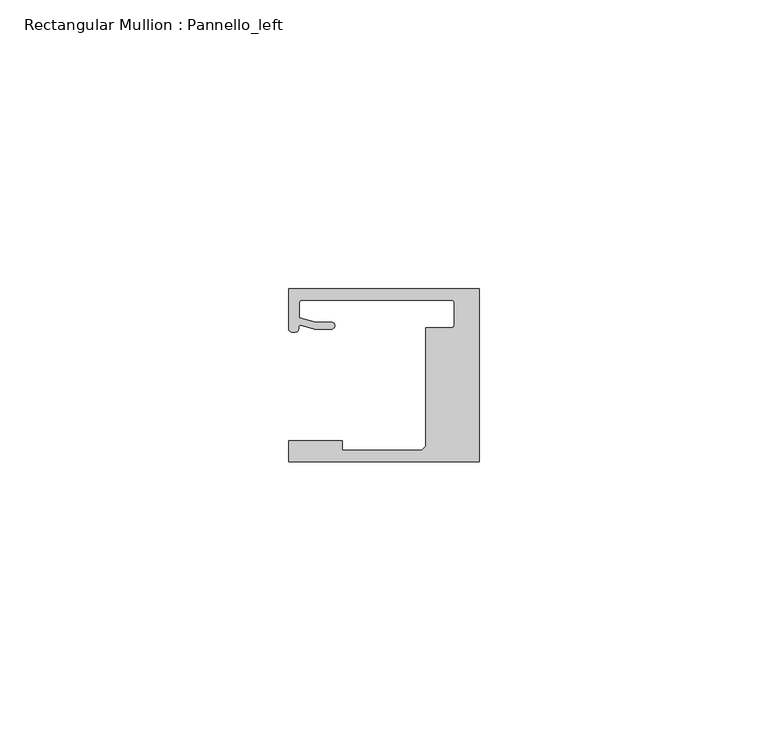
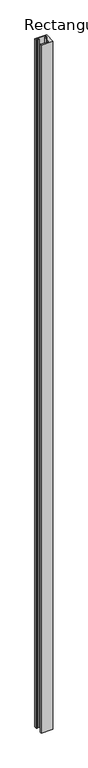
"""IFC4 building model written with IfcOpenShell, lengths in millimetres: member geometry, Rectangular Mullion : Pannello_left."""

from ifc_helpers import new_model, si_unit, frame, origin, place, context, project, spatial, polyline, circle_curve, source, transform, mapped, element, save
from ifc_brep_helpers import plane_surface, cylinder_surface, revolved_surface, extruded_surface, spline_curve, advanced_brep


def rectangular_mullion_pannello_left_b0e93784(model_context):
    return source(origin(), model_context, "Body", "AdvancedBrep", [
        advanced_brep(
        [(-33.0, -15.0, 0.0), (0.0, -15.0, 0.0), (0.0, 15.0, 0.0), (-33.0000135, 15.0, 0.0), (-33.0000135, 8.0000472, 0.0), (-30.9223017, 8.6490241, 0.0), (-28.4999305, 7.9999523, 0.0), (-25.59998, 7.9999523, 0.0), (-25.59998, 9.1999523, 0.0), (-28.3419477, 9.1999523, 0.0), (-31.19998, 9.9657591, 0.0), (-31.19998, 12.50001, 0.0), (-30.69998, 13.00001, 0.0), (-4.7999726, 13.00001, 0.0), (-4.2999726, 12.50001, 0.0), (-4.2999726, 8.7500595, 0.0), (-4.7999726, 8.2500595, 0.0), (-9.2999726, 8.2500595, 0.0), (-9.2999726, -12.2999849, 0.0), (-10.0000103, -13.0000004, 0.0), (-23.700041, -13.0000004, 0.0), (-23.700041, -11.3000004, 0.0), (-33.0, -11.3000004, 0.0), (-33.0, -15.0, -2026.9999865), (-33.0, -11.3000004, -2026.9999865), (-23.700041, -11.3000004, -2026.9999865), (-23.700041, -13.0000004, -2026.9999865), (-10.0000103, -13.0000004, -2026.9999865), (-9.2999726, -12.2999849, -2026.9999865), (-9.2999726, 8.2500595, -2026.9999865), (-4.7999726, 8.2500595, -2026.9999865), (-4.2999726, 8.7500595, -2026.9999865), (-4.2999726, 12.50001, -2026.9999865), (-4.7999726, 13.00001, -2026.9999865), (-30.69998, 13.00001, -2026.9999865), (-31.19998, 12.50001, -2026.9999865), (-31.19998, 9.9657591, -2026.9999865), (-28.3419477, 9.1999523, -2026.9999865), (-25.59998, 9.1999523, -2026.9999865), (-25.59998, 7.9999523, -2026.9999865), (-28.4999305, 7.9999523, -2026.9999865), (-30.9223017, 8.6490241, -2026.9999865), (-33.0000135, 8.0000472, -2026.9999865), (-33.0000135, 15.0, -2026.9999865), (0.0, 15.0, -2026.9999865), (0.0, -15.0, -2026.9999865)],
        [
            (0, 1),
            (1, 2),
            (2, 3),
            (3, 4),
            (4, 5, spline_curve(3, [(-33.0000135, 8.0000472, 0.0), (-33.0000135, 7.457047519, 0.0), (-32.262327879, 7.456527435, 0.0), (-31.357433266, 7.563996614, 0.0), (-31.305645054, 7.690065204, 0.0), (-31.298563602, 8.366228555, 0.0), (-31.312054066, 8.717747958, 0.0), (-30.9223017, 8.6490241, 0.0)], [4, 2, 2, 4], [0.0, 0.0027053965905959043, 0.0058611956533709, 0.007702013405570312])),
            (5, 6),
            (6, 7),
            (7, 8, circle_curve(frame((-25.59998, 8.5999523, 0.0), z_axis=(0.0, 0.0, 1.0), x_axis=(0.0, 1.0, 0.0)), 0.6)),
            (8, 9),
            (9, 10),
            (10, 11),
            (11, 12, circle_curve(frame((-30.69998, 12.50001, 0.0), z_axis=(0.0, 0.0, -1.0), x_axis=(0.0, 1.0, 0.0)), 0.5)),
            (12, 13),
            (13, 14, circle_curve(frame((-4.7999726, 12.50001, 0.0), z_axis=(0.0, 0.0, -1.0), x_axis=(1.0, 0.0, 0.0)), 0.5)),
            (14, 15),
            (15, 16, circle_curve(frame((-4.7999726, 8.7500595, 0.0), z_axis=(0.0, 0.0, -1.0), x_axis=(0.0, -1.0, 0.0)), 0.5)),
            (16, 17),
            (17, 18),
            (18, 19),
            (19, 20),
            (20, 21),
            (21, 22),
            (22, 0),
            (23, 24),
            (24, 25),
            (25, 26),
            (26, 27),
            (27, 28),
            (28, 29),
            (29, 30),
            (30, 31, circle_curve(frame((-4.7999726, 8.7500595, -2026.9999865), z_axis=(0.0, 0.0, 1.0), x_axis=(0.0, -1.0, 0.0)), 0.5)),
            (31, 32),
            (32, 33, circle_curve(frame((-4.7999726, 12.50001, -2026.9999865), z_axis=(0.0, 0.0, 1.0), x_axis=(1.0, 0.0, 0.0)), 0.5)),
            (33, 34),
            (34, 35, circle_curve(frame((-30.69998, 12.50001, -2026.9999865), z_axis=(0.0, 0.0, 1.0), x_axis=(0.0, 1.0, 0.0)), 0.5)),
            (35, 36),
            (36, 37),
            (37, 38),
            (38, 39, circle_curve(frame((-25.59998, 8.5999523, -2026.9999865), z_axis=(0.0, 0.0, -1.0), x_axis=(0.0, 1.0, 0.0)), 0.6)),
            (39, 40),
            (40, 41),
            (41, 42, spline_curve(3, [(-30.9223017, 8.6490241, -2026.9999865), (-31.312054066, 8.717747958, -2026.9999865), (-31.298563602, 8.366228555, -2026.9999865), (-31.305645054, 7.690065204, -2026.9999865), (-31.357433266, 7.563996614, -2026.9999865), (-32.262327879, 7.456527435, -2026.9999865), (-33.0000135, 7.457047519, -2026.9999865), (-33.0000135, 8.0000472, -2026.9999865)], [4, 2, 2, 4], [0.0, 0.001840817752199412, 0.004996616814974408, 0.007702013405570312])),
            (42, 43),
            (43, 44),
            (44, 45),
            (45, 23),
            (0, 23),
            (45, 1),
            (44, 2),
            (43, 3),
            (42, 4),
            (41, 5),
            (40, 6),
            (39, 7),
            (38, 8),
            (37, 9),
            (36, 10),
            (35, 11),
            (34, 12),
            (33, 13),
            (32, 14),
            (31, 15),
            (30, 16),
            (29, 17),
            (28, 18),
            (27, 19),
            (26, 20),
            (25, 21),
            (24, 22),
        ],
        [
            plane_surface(frame((0.0, -36.2491502, 0.0), z_axis=(0.0, 0.0, 1.0), x_axis=(-1.0, 0.0, 0.0))),
            plane_surface(frame((0.0, -36.2491502, -2026.9999865), z_axis=(0.0, 0.0, -1.0), x_axis=(-1.0, 0.0, 0.0))),
            plane_surface(frame((-33.0, -15.0, 0.0), z_axis=(0.0, -1.0, 0.0), x_axis=(0.0, 0.0, -1.0))),
            plane_surface(frame((0.0, -15.0, 0.0), z_axis=(1.0, 0.0, 0.0), x_axis=(0.0, 0.0, -1.0))),
            plane_surface(frame((0.0, 15.0, 0.0), z_axis=(0.0, 1.0, 0.0), x_axis=(0.0, 0.0, -1.0))),
            plane_surface(frame((-33.0000135, 15.0, 0.0), z_axis=(-1.0, 0.0, 0.0), x_axis=(0.0, 0.0, -1.0))),
            extruded_surface(spline_curve(3, [(-33.0000135, 8.0000472, -2026.9999865), (-33.0000135, 7.457047519, -2026.9999865), (-32.262327879, 7.456527435, -2026.9999865), (-31.357433266, 7.563996614, -2026.9999865), (-31.305645054, 7.690065204, -2026.9999865), (-31.298563602, 8.366228555, -2026.9999865), (-31.312054066, 8.717747958, -2026.9999865), (-30.9223017, 8.6490241, -2026.9999865)], [4, 2, 2, 4], [0.0, 0.0027053965905959043, 0.0058611956533709, 0.007702013405570312]), (0.0, 0.0, 2026.9999865), 2026.9999865),
            plane_surface(frame((-30.9223017, 8.6490241, 0.0), z_axis=(-0.25881883200192934, -0.9659258833891746, 0.0), x_axis=(0.0, 0.0, -1.0))),
            plane_surface(frame((-28.4999305, 7.9999523, 0.0), z_axis=(0.0, -1.0, 0.0), x_axis=(0.0, 0.0, -1.0))),
            cylinder_surface(frame((-25.59998, 8.5999523, 0.0), z_axis=(0.0, 0.0, 1.0), x_axis=(0.0, 1.0, 0.0)), 0.6),
            plane_surface(frame((-25.59998, 9.1999523, 0.0), z_axis=(0.0, 1.0, 0.0), x_axis=(0.0, 0.0, -1.0))),
            plane_surface(frame((-28.3419477, 9.1999523, 0.0), z_axis=(0.25881883204288636, 0.9659258833782002, 0.0), x_axis=(0.0, 0.0, -1.0))),
            plane_surface(frame((-31.19998, 9.9657591, 0.0), z_axis=(1.0, 0.0, 0.0), x_axis=(0.0, 0.0, -1.0))),
            revolved_surface(polyline([(-30.69998, 13.00001, -2026.9999865), (-30.69998, 13.00001, 0.0)]), (-30.69998, 12.50001, 0.0), (0.0, 0.0, -1.0)),
            plane_surface(frame((-30.69998, 13.00001, 0.0), z_axis=(0.0, -1.0, 0.0), x_axis=(0.0, 0.0, -1.0))),
            revolved_surface(polyline([(-4.2999726, 12.50001, -2026.9999865), (-4.2999726, 12.50001, 0.0)]), (-4.7999726, 12.50001, 0.0), (0.0, 0.0, -1.0)),
            plane_surface(frame((-4.2999726, 12.50001, 0.0), z_axis=(-1.0, 0.0, 0.0), x_axis=(0.0, 0.0, -1.0))),
            revolved_surface(polyline([(-4.7999726, 8.2500595, -2026.9999865), (-4.7999726, 8.2500595, 0.0)]), (-4.7999726, 8.7500595, 0.0), (0.0, 0.0, -1.0)),
            plane_surface(frame((-4.7999726, 8.2500595, 0.0), z_axis=(0.0, 1.0, 0.0), x_axis=(0.0, 0.0, -1.0))),
            plane_surface(frame((-9.2999726, 8.2500595, 0.0), z_axis=(-1.0, 0.0, 0.0), x_axis=(0.0, 0.0, -1.0))),
            plane_surface(frame((-9.2999726, -12.2999849, 0.0), z_axis=(-0.7070955486277984, 0.7071180135668678, 0.0), x_axis=(0.0, 0.0, -1.0))),
            plane_surface(frame((-10.0000103, -13.0000004, 0.0), z_axis=(0.0, 1.0, 0.0), x_axis=(0.0, 0.0, -1.0))),
            plane_surface(frame((-23.700041, -13.0000004, 0.0), z_axis=(1.0, 0.0, 0.0), x_axis=(0.0, 0.0, -1.0))),
            plane_surface(frame((-23.700041, -11.3000004, 0.0), z_axis=(0.0, 1.0, 0.0), x_axis=(0.0, 0.0, -1.0))),
            plane_surface(frame((-33.0, -11.3000004, 0.0), z_axis=(-1.0, 0.0, 0.0), x_axis=(0.0, 0.0, -1.0))),
        ],
        [
            (0, [[1, 2, 3, 4, 5, 6, 7, 8, 9, 10, 11, 12, 13, 14, 15, 16, 17, 18, 19, 20, 21, 22, 23]]),
            (1, [[24, 25, 26, 27, 28, 29, 30, 31, 32, 33, 34, 35, 36, 37, 38, 39, 40, 41, 42, 43, 44, 45, 46]]),
            (2, [[-1, 47, -46, 48]]),
            (3, [[-2, -48, -45, 49]]),
            (4, [[-3, -49, -44, 50]]),
            (5, [[-4, -50, -43, 51]]),
            (6, [[-5, -51, -42, 52]]),
            (7, [[-6, -52, -41, 53]]),
            (8, [[-7, -53, -40, 54]]),
            (9, [[-8, -54, -39, 55]]),
            (10, [[-9, -55, -38, 56]]),
            (11, [[-10, -56, -37, 57]]),
            (12, [[-11, -57, -36, 58]]),
            (13, [[-12, -58, -35, 59]]),
            (14, [[-13, -59, -34, 60]]),
            (15, [[-14, -60, -33, 61]]),
            (16, [[-15, -61, -32, 62]]),
            (17, [[-16, -62, -31, 63]]),
            (18, [[-17, -63, -30, 64]]),
            (19, [[-18, -64, -29, 65]]),
            (20, [[-19, -65, -28, 66]]),
            (21, [[-20, -66, -27, 67]]),
            (22, [[-21, -67, -26, 68]]),
            (23, [[-22, -68, -25, 69]]),
            (24, [[-23, -69, -24, -47]]),
        ],
    ),
    ])


if __name__ == "__main__":
    model = new_model("IFC4")
    model_context = context("Model", 3, world=origin())
    ifc_project = project(units=[si_unit("LENGTHUNIT", "METRE", prefix="MILLI")], contexts=[model_context])
    site = spatial("IfcSite", under=ifc_project)
    building = spatial("IfcBuilding", under=site)
    placement = place(None, origin())
    rectangular_mullion_pannello_left_shape = rectangular_mullion_pannello_left_b0e93784(model_context)
    element("IfcMember", 1, ObjectType="Rectangular Mullion : Pannello_left", at=placement, inside=building, context=model_context, shape_type="MappedRepresentation", body=[
        mapped(rectangular_mullion_pannello_left_shape, transform((0.0, 0.0, 0.0), x_axis=(1.0, 0.0, 0.0), y_axis=(0.0, 1.0, 0.0), z_axis=(0.0, 0.0, 1.0))),
    ])
    save(model, "model.ifc")

# Revit data of these elements
# Type "Rectangular Mullion : Pannello_left"
#   built-in parameter 1007322 = 0.0984252 (stored number, unit not read)
#   built-in parameter 1007320 = 0.0305117 (stored number, unit not read)
